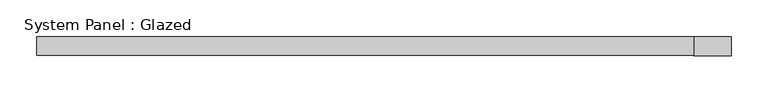
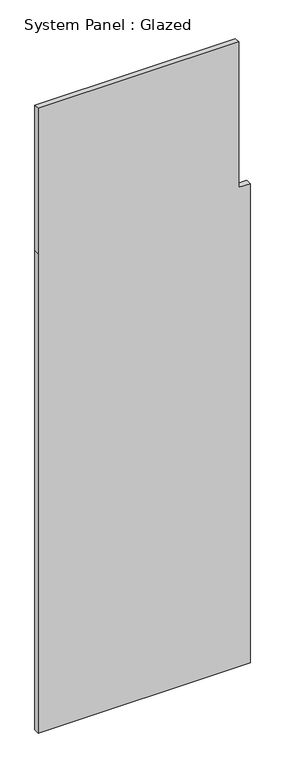
"""IFC4 building model written with IfcOpenShell, lengths in millimetres: plate geometry, System Panel : Glazed."""

from ifc_helpers import new_model, si_unit, frame, origin, place, context, project, spatial, polyline, outline, extrude, source, transform, mapped, element, save


def system_panel_glazed_562398b4(model_context):
    return source(origin(), model_context, "Body", "SweptSolid", [
        extrude(outline(polyline([(0.0, -472.4310996), (0.0, 472.4310996), (2260.6, 472.4310996), (2260.6, 421.6310996), (2946.4, 421.6310996), (2946.4, -472.4310996), (2260.6, -472.4310996), (0.0, -472.4310996)])), frame((0.0, -12.7, 0.0), z_axis=(0.0, 1.0, 0.0), x_axis=(0.0, 0.0, 1.0)), (0.0, 0.0, 1.0), 25.4),
    ])


if __name__ == "__main__":
    model = new_model("IFC4")
    model_context = context("Model", 3, world=origin())
    ifc_project = project(units=[si_unit("LENGTHUNIT", "METRE", prefix="MILLI")], contexts=[model_context])
    site = spatial("IfcSite", under=ifc_project)
    building = spatial("IfcBuilding", under=site)
    placement = place(None, origin())
    system_panel_glazed_shape = system_panel_glazed_562398b4(model_context)
    element("IfcPlate", 1, ObjectType="System Panel : Glazed", at=placement, inside=building, context=model_context, shape_type="MappedRepresentation", body=[
        mapped(system_panel_glazed_shape, transform((0.0, 0.0, 0.0), x_axis=(1.0, 0.0, 0.0), y_axis=(0.0, 1.0, 0.0), z_axis=(0.0, 0.0, 1.0))),
    ])
    save(model, "model.ifc")

# Revit data of these elements
# Element 1 (IfcPlate, "System Panel : Glazed")
#   Materials on its faces: "BUTT GLAZED STOREFRONT WITH VERTICAL MULLION"
# Materials
#   "BUTT GLAZED STOREFRONT WITH VERTICAL MULLION": class "Glass", colour RGB 236 240 239, transparency 0.39, Description = "Soda Lime Glass", Cost = 0
